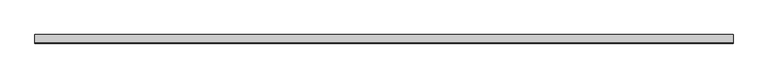
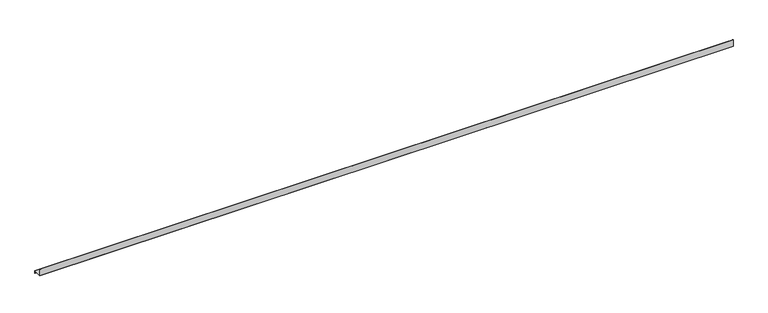
"""IFC4 building model written with IfcOpenShell, lengths in millimetres: proxy geometry, Generic Models 3:Generic Models 2:312240:Generic Models 2:312240 : Generic Models 3:Generic Models 2:312240:10 : Generic Models 3:Generic Models 2:312240:Generic Models 2:312240 : Generic Models 3:Generic Models 2:312240:300533."""

from ifc_helpers import new_model, si_unit, frame, origin, place, context, project, spatial, polyline, outline, extrude, source, transform, mapped, element, save


def generic_models_e09d9f95(model_context):
    return source(origin(), model_context, "Body", "SweptSolid", [
        extrude(outline(polyline([(-530573.5923718, -47.625), (-530573.5923718, -38.1), (-530572.7986218, -38.1), (-530572.7986218, -46.83125), (-530569.6236218, -46.83125), (-530569.6236218, -26.19375), (-530645.4413841, -26.19375), (-530645.4413841, 33.2475906), (-530644.6476341, 33.2475906), (-530644.6476341, -25.4), (-530568.8298718, -25.4), (-530568.8298718, -47.625), (-530573.5923718, -47.625)])), frame((560221.5370374, 0.0, 0.0), z_axis=(1.0, 0.0, 0.0), x_axis=(0.0, 1.0, 0.0)), (0.0, 0.0, 1.0), 6194.1576562),
    ])


if __name__ == "__main__":
    model = new_model("IFC4")
    model_context = context("Model", 3, world=origin())
    ifc_project = project(units=[si_unit("LENGTHUNIT", "METRE", prefix="MILLI")], contexts=[model_context])
    site = spatial("IfcSite", under=ifc_project)
    building = spatial("IfcBuilding", under=site)
    placement = place(None, origin())
    generic_models_shape = generic_models_e09d9f95(model_context)
    element("IfcBuildingElementProxy", 1, Name="Generic Models 3:Generic Models 2:312240:Generic Models 2:312240 : Generic Models 3:Generic Models 2:312240:10 : Generic Models 3:Generic Models 2:312240:Generic Models 2:312240 : Generic Models 3:Generic Models 2:312240:300533", ObjectType="Generic Models 3:Generic Models 2:312240:Generic Models 2:312240 : Generic Models 3:Generic Models 2:312240:10 : Generic Models 3:Generic Models 2:312240:Generic Models 2:312240 : Generic Models 3:Generic Models 2:312240:300533", at=placement, inside=building, context=model_context, shape_type="MappedRepresentation", body=[
        mapped(generic_models_shape, transform((0.0, 0.0, 0.0), x_axis=(1.0, 0.0, 0.0), y_axis=(0.0, 1.0, 0.0), z_axis=(0.0, 0.0, 1.0))),
    ])
    save(model, "model.ifc")

# Revit data of these elements
# Type "Generic Models 3:Generic Models 2:312240:Generic Models 2:312240 : Generic Models 3:Generic Models 2:312240:10 : Generic Models 3:Generic Models 2:312240:Generic Models 2:312240 : Generic Models 3:Generic Models 2:312240:300533"
#   NameOverride = "Generic Models 3:Generic Models 2:312240:Generic Models 2:312240 : Generic Models 3:Generic Models 2:312240:300533"
#   ObjectTypeOverride = "Generic Models 2:312240 : Generic Models 3:Generic Models 2:312240"
#   Reference = "Generic Models 2"
#   Tag = "300533"
# Element 1 (IfcBuildingElementProxy, "Generic Models 3:Generic Models 2:312240:Generic Models 2:312240 : Generic Models 3:Generic Models 2:312240:10 : Generic Models 3:Generic Models 2:312240:Generic Models 2:312240 : Generic Models 3:Generic Models 2:312240:300533")
#   Materials on its faces: "BRAKE METAL FLASHING WITH BACK & END DAMS"
# Materials
#   "BRAKE METAL FLASHING WITH BACK & END DAMS": class "Unassigned", colour RGB 182 182 182, transparency 0, Cost = 0
